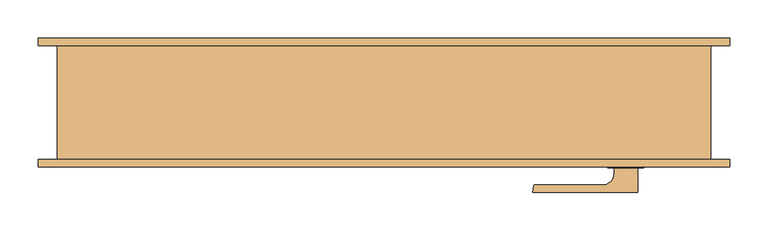
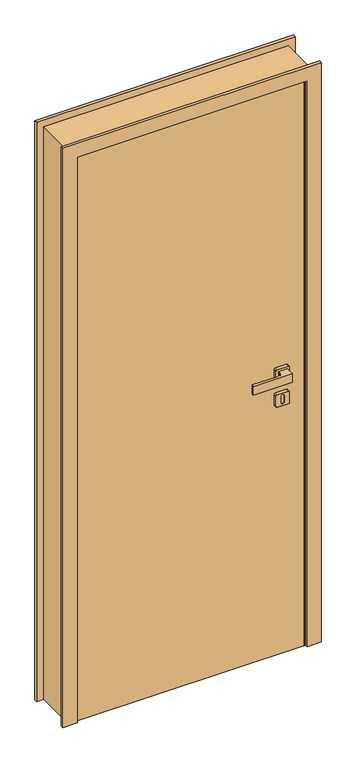
"""IFC4 building model written with IfcOpenShell, lengths in millimetres: door geometry, porta multiplas_growarq : porta giro simples 80 cm_growarq 2."""

from ifc_helpers import new_model, si_unit, point, frame, frame_2d, origin, origin_with_axes, place, context, project, spatial, polyline, circle_curve, trimmed, segment, composite_curve, outline, extrude, source, transform, mapped, element, save
from ifc_brep_helpers import plane_surface, cylinder_surface, revolved_surface, advanced_brep


def door_ea212285(model_context):
    return source(origin(), model_context, "Body", "SolidModel", [
        advanced_brep(
        [(337.5247906, -86.0, 975.2140175), (298.4820692, -86.0, 975.2140175), (294.475196, -86.0, 971.2071442), (294.475196, -86.0, 932.3348635), (298.475196, -86.0, 928.3348635), (337.5247906, -86.0, 928.3348635), (341.5247906, -86.0, 932.3348635), (341.5247906, -86.0, 971.2140175), (323.0036235, -86.0, 963.1453546), (323.0036235, -86.0, 940.4035264), (312.9935514, -86.0, 940.4035264), (312.9935514, -86.0, 963.1453546), (337.5247906, -75.0, 975.2140175), (341.5247906, -75.0, 971.2140175), (341.5247906, -75.0, 932.3348635), (337.5247906, -75.0, 928.3348635), (298.475196, -75.0, 928.3348635), (294.475196, -75.0, 932.3348635), (294.475196, -75.0, 971.2071442), (298.4820692, -75.0, 975.2140175), (323.0036235, -84.0, 940.4035264), (323.0036235, -84.0, 963.1453546), (312.9935514, -84.0, 963.1453546), (312.9935514, -84.0, 940.4035264)],
        [
            (0, 1),
            (1, 2, circle_curve(frame((298.4820692, -86.0, 971.2071442), z_axis=(0.0, -1.0, 0.0), x_axis=(1.0, 0.0, 0.0)), 4.0068732)),
            (2, 3),
            (3, 4, circle_curve(frame((298.475196, -86.0, 932.3348635), z_axis=(0.0, -1.0, 0.0), x_axis=(1.0, 0.0, 0.0)), 4.0)),
            (4, 5),
            (5, 6, circle_curve(frame((337.5247906, -86.0, 932.3348635), z_axis=(0.0, -1.0, 0.0), x_axis=(1.0, 0.0, 0.0)), 4.0)),
            (6, 7),
            (7, 0, circle_curve(frame((337.5247906, -86.0, 971.2140175), z_axis=(0.0, -1.0, 0.0), x_axis=(1.0, 0.0, 0.0)), 4.0)),
            (8, 9),
            (9, 10, circle_curve(frame((317.9985874, -86.0, 940.4035264), z_axis=(0.0, 1.0, 0.0), x_axis=(1.0, 0.0, 0.0)), 5.0050361)),
            (10, 11),
            (11, 8, circle_curve(frame((317.9985874, -86.0, 963.1453546), z_axis=(0.0, 1.0, 0.0), x_axis=(1.0, 0.0, 0.0)), 5.0050361)),
            (12, 13, circle_curve(frame((337.5247906, -75.0, 971.2140175), z_axis=(0.0, 1.0, 0.0), x_axis=(1.0, 0.0, 0.0)), 4.0)),
            (13, 14),
            (14, 15, circle_curve(frame((337.5247906, -75.0, 932.3348635), z_axis=(0.0, 1.0, 0.0), x_axis=(1.0, 0.0, 0.0)), 4.0)),
            (15, 16),
            (16, 17, circle_curve(frame((298.475196, -75.0, 932.3348635), z_axis=(0.0, 1.0, 0.0), x_axis=(1.0, 0.0, 0.0)), 4.0)),
            (17, 18),
            (18, 19, circle_curve(frame((298.4820692, -75.0, 971.2071442), z_axis=(0.0, 1.0, 0.0), x_axis=(1.0, 0.0, 0.0)), 4.0068732)),
            (19, 12),
            (0, 12),
            (19, 1),
            (18, 2),
            (17, 3),
            (16, 4),
            (15, 5),
            (14, 6),
            (13, 7),
            (20, 21),
            (21, 22, circle_curve(frame((317.9985874, -84.0, 963.1453546), z_axis=(0.0, -1.0, 0.0), x_axis=(1.0, 0.0, 0.0)), 5.0050361)),
            (22, 23),
            (23, 20, circle_curve(frame((317.9985874, -84.0, 940.4035264), z_axis=(0.0, -1.0, 0.0), x_axis=(1.0, 0.0, 0.0)), 5.0050361)),
            (20, 9),
            (8, 21),
            (22, 11),
            (10, 23),
        ],
        [
            plane_surface(frame((298.4781039, -86.0, 975.2140175), z_axis=(0.0, -1.0, 0.0), x_axis=(-1.0, 0.0, 0.0))),
            plane_surface(frame((298.4781039, -75.0, 975.2140175), z_axis=(0.0, 1.0, 0.0), x_axis=(1.0, 0.0, 0.0))),
            plane_surface(frame((337.5247906, -86.0, 975.2140175), z_axis=(0.0, 0.0, 1.0), x_axis=(0.0, 1.0, 0.0))),
            cylinder_surface(frame((298.4820692, -75.0, 971.2071442), z_axis=(0.0, -1.0, 0.0), x_axis=(1.0, 0.0, 0.0)), 4.0068732),
            plane_surface(frame((294.475196, -86.0, 971.2071442), z_axis=(-1.0, 0.0, 0.0), x_axis=(0.0, 1.0, 0.0))),
            cylinder_surface(frame((298.475196, -75.0, 932.3348635), z_axis=(0.0, -1.0, 0.0), x_axis=(1.0, 0.0, 0.0)), 4.0),
            plane_surface(frame((298.475196, -86.0, 928.3348635), z_axis=(0.0, 0.0, -1.0), x_axis=(0.0, 1.0, 0.0))),
            cylinder_surface(frame((337.5247906, -75.0, 932.3348635), z_axis=(0.0, -1.0, 0.0), x_axis=(1.0, 0.0, 0.0)), 4.0),
            plane_surface(frame((341.5247906, -86.0, 932.3348635), z_axis=(1.0, 0.0, 0.0), x_axis=(0.0, 1.0, 0.0))),
            cylinder_surface(frame((337.5247906, -75.0, 971.2140175), z_axis=(0.0, -1.0, 0.0), x_axis=(1.0, 0.0, 0.0)), 4.0),
            plane_surface(frame((323.0036235, -84.0, 952.9958878), z_axis=(0.0, -1.0, 0.0), x_axis=(0.0, 0.0, -1.0))),
            plane_surface(frame((323.0036235, -86.0, 940.4035264), z_axis=(-1.0, 0.0, 0.0), x_axis=(0.0, 1.0, 0.0))),
            plane_surface(frame((312.9935514, -86.0, 963.1453546), z_axis=(1.0, 0.0, 0.0), x_axis=(0.0, 1.0, 0.0))),
            revolved_surface(polyline([(323.0036235, -86.0, 940.4035264), (323.0036235, -84.0, 940.4035264)]), (317.9985874, -84.0, 940.4035264), (0.0, -1.0, 0.0)),
            revolved_surface(polyline([(323.0036235, -86.0, 963.1453546), (323.0036235, -84.0, 963.1453546)]), (317.9985874, -84.0, 963.1453546), (0.0, -1.0, 0.0)),
        ],
        [
            (0, [[1, 2, 3, 4, 5, 6, 7, 8], [9, 10, 11, 12]]),
            (1, [[13, 14, 15, 16, 17, 18, 19, 20]]),
            (2, [[-1, 21, -20, 22]]),
            (3, [[-2, -22, -19, 23]]),
            (4, [[-3, -23, -18, 24]]),
            (5, [[-4, -24, -17, 25]]),
            (6, [[-5, -25, -16, 26]]),
            (7, [[-6, -26, -15, 27]]),
            (8, [[-7, -27, -14, 28]]),
            (9, [[-8, -28, -13, -21]]),
            (10, [[29, 30, 31, 32]]),
            (11, [[-29, 33, -9, 34]]),
            (12, [[-31, 35, -11, 36]]),
            (13, [[-32, -36, -10, -33]]),
            (14, [[-30, -34, -12, -35]]),
        ],
    ),
        advanced_brep(
        [(337.5247906, -86.0, 1068.227973), (298.4820692, -86.0, 1068.227973), (294.475196, -86.0, 1064.2210998), (294.475196, -86.0, 1025.3488191), (298.475196, -86.0, 1021.3488191), (337.5247906, -86.0, 1021.3488191), (341.5247906, -86.0, 1025.3488191), (341.5247906, -86.0, 1064.227973), (337.5247906, -75.0, 1068.227973), (341.5247906, -75.0, 1064.227973), (341.5247906, -75.0, 1025.3488191), (337.5247906, -75.0, 1021.3488191), (298.475196, -75.0, 1021.3488191), (294.475196, -75.0, 1025.3488191), (294.475196, -75.0, 1064.2210998), (298.4820692, -75.0, 1068.227973)],
        [
            (0, 1),
            (1, 2, circle_curve(frame((298.4820692, -86.0, 1064.2210998), z_axis=(0.0, -1.0, 0.0), x_axis=(1.0, 0.0, 0.0)), 4.0068732)),
            (2, 3),
            (3, 4, circle_curve(frame((298.475196, -86.0, 1025.3488191), z_axis=(0.0, -1.0, 0.0), x_axis=(1.0, 0.0, 0.0)), 4.0)),
            (4, 5),
            (5, 6, circle_curve(frame((337.5247906, -86.0, 1025.3488191), z_axis=(0.0, -1.0, 0.0), x_axis=(1.0, 0.0, 0.0)), 4.0)),
            (6, 7),
            (7, 0, circle_curve(frame((337.5247906, -86.0, 1064.227973), z_axis=(0.0, -1.0, 0.0), x_axis=(1.0, 0.0, 0.0)), 4.0)),
            (8, 9, circle_curve(frame((337.5247906, -75.0, 1064.227973), z_axis=(0.0, 1.0, 0.0), x_axis=(1.0, 0.0, 0.0)), 4.0)),
            (9, 10),
            (10, 11, circle_curve(frame((337.5247906, -75.0, 1025.3488191), z_axis=(0.0, 1.0, 0.0), x_axis=(1.0, 0.0, 0.0)), 4.0)),
            (11, 12),
            (12, 13, circle_curve(frame((298.475196, -75.0, 1025.3488191), z_axis=(0.0, 1.0, 0.0), x_axis=(1.0, 0.0, 0.0)), 4.0)),
            (13, 14),
            (14, 15, circle_curve(frame((298.4820692, -75.0, 1064.2210998), z_axis=(0.0, 1.0, 0.0), x_axis=(1.0, 0.0, 0.0)), 4.0068732)),
            (15, 8),
            (0, 8),
            (15, 1),
            (14, 2),
            (13, 3),
            (12, 4),
            (11, 5),
            (10, 6),
            (9, 7),
        ],
        [
            plane_surface(frame((298.4781039, -86.0, 975.2140175), z_axis=(0.0, -1.0, 0.0), x_axis=(-1.0, 0.0, 0.0))),
            plane_surface(frame((298.4781039, -75.0, 975.2140175), z_axis=(0.0, 1.0, 0.0), x_axis=(1.0, 0.0, 0.0))),
            plane_surface(frame((337.5247906, -86.0, 1068.227973), z_axis=(0.0, 0.0, 1.0), x_axis=(0.0, 1.0, 0.0))),
            cylinder_surface(frame((298.4820692, -75.0, 1064.2210998), z_axis=(0.0, -1.0, 0.0), x_axis=(1.0, 0.0, 0.0)), 4.0068732),
            plane_surface(frame((294.475196, -86.0, 1064.2210998), z_axis=(-1.0, 0.0, 0.0), x_axis=(0.0, 1.0, 0.0))),
            cylinder_surface(frame((298.475196, -75.0, 1025.3488191), z_axis=(0.0, -1.0, 0.0), x_axis=(1.0, 0.0, 0.0)), 4.0),
            plane_surface(frame((298.475196, -86.0, 1021.3488191), z_axis=(0.0, 0.0, -1.0), x_axis=(0.0, 1.0, 0.0))),
            cylinder_surface(frame((337.5247906, -75.0, 1025.3488191), z_axis=(0.0, -1.0, 0.0), x_axis=(1.0, 0.0, 0.0)), 4.0),
            plane_surface(frame((341.5247906, -86.0, 1025.3488191), z_axis=(1.0, 0.0, 0.0), x_axis=(0.0, 1.0, 0.0))),
            cylinder_surface(frame((337.5247906, -75.0, 1064.227973), z_axis=(0.0, -1.0, 0.0), x_axis=(1.0, 0.0, 0.0)), 4.0),
        ],
        [
            (0, [[1, 2, 3, 4, 5, 6, 7, 8]]),
            (1, [[9, 10, 11, 12, 13, 14, 15, 16]]),
            (2, [[-1, 17, -16, 18]]),
            (3, [[-2, -18, -15, 19]]),
            (4, [[-3, -19, -14, 20]]),
            (5, [[-4, -20, -13, 21]]),
            (6, [[-5, -21, -12, 22]]),
            (7, [[-6, -22, -11, 23]]),
            (8, [[-7, -23, -10, 24]]),
            (9, [[-8, -24, -9, -17]]),
        ],
    ),
        extrude(outline(composite_curve([segment(polyline([(333.5247906, -118.5150355), (195.5657525, -118.5150355), (197.1621392, -109.4614767)]), True, "CONTINUOUS"), segment(trimmed(circle_curve(frame_2d((198.1590205, -109.6372538)), 1.0122598), [point((197.1621392, -109.4614767))], [point((198.1590205, -108.6249939))], False, "CARTESIAN"), True, "CONTINUOUS"), segment(polyline([(198.1590205, -108.6249939), (287.4483579, -108.6249939)]), True, "CONTINUOUS"), segment(trimmed(circle_curve(frame_2d((287.4483579, -93.5981558)), 15.0268381), [point((287.4483579, -108.6249939))], [point((302.475196, -93.5981558))], True, "CARTESIAN"), True, "CONTINUOUS"), segment(polyline([(302.475196, -93.5981558), (302.475196, -86.7793682), (333.5247906, -86.7793682), (333.5247906, -118.5150355)]), True, "CONTINUOUS")], self_intersect=False)), frame((0.0, 0.0, 1029.3488191), z_axis=(0.0, 0.0, 1.0), x_axis=(1.0, 0.0, 0.0)), (0.0, 0.0, 1.0), 30.8791539),
        advanced_brep(
        [(337.5247906, -34.0, 975.2140175), (341.5247906, -34.0, 971.2140175), (341.5247906, -34.0, 932.3348635), (337.5247906, -34.0, 928.3348635), (298.475196, -34.0, 928.3348635), (294.475196, -34.0, 932.3348635), (294.475196, -34.0, 971.2071442), (298.4820692, -34.0, 975.2140175), (323.0036235, -34.0, 963.1453546), (312.9935514, -34.0, 963.1453546), (312.9935514, -34.0, 940.4035264), (323.0036235, -34.0, 940.4035264), (337.5247906, -45.0, 975.2140175), (298.4820692, -45.0, 975.2140175), (294.475196, -45.0, 971.2071442), (294.475196, -45.0, 932.3348635), (298.475196, -45.0, 928.3348635), (337.5247906, -45.0, 928.3348635), (341.5247906, -45.0, 932.3348635), (341.5247906, -45.0, 971.2140175), (323.0036235, -36.0, 940.4035264), (312.9935514, -36.0, 940.4035264), (312.9935514, -36.0, 963.1453546), (323.0036235, -36.0, 963.1453546)],
        [
            (0, 1, circle_curve(frame((337.5247906, -34.0, 971.2140175), z_axis=(0.0, 1.0, 0.0), x_axis=(1.0, 0.0, 0.0)), 4.0)),
            (1, 2),
            (2, 3, circle_curve(frame((337.5247906, -34.0, 932.3348635), z_axis=(0.0, 1.0, 0.0), x_axis=(1.0, 0.0, 0.0)), 4.0)),
            (3, 4),
            (4, 5, circle_curve(frame((298.475196, -34.0, 932.3348635), z_axis=(0.0, 1.0, 0.0), x_axis=(1.0, 0.0, 0.0)), 4.0)),
            (5, 6),
            (6, 7, circle_curve(frame((298.4820692, -34.0, 971.2071442), z_axis=(0.0, 1.0, 0.0), x_axis=(1.0, 0.0, 0.0)), 4.0068732)),
            (7, 0),
            (8, 9, circle_curve(frame((317.9985874, -34.0, 963.1453546), z_axis=(0.0, -1.0, 0.0), x_axis=(1.0, 0.0, 0.0)), 5.0050361)),
            (9, 10),
            (10, 11, circle_curve(frame((317.9985874, -34.0, 940.4035264), z_axis=(0.0, -1.0, 0.0), x_axis=(1.0, 0.0, 0.0)), 5.0050361)),
            (11, 8),
            (12, 13),
            (13, 14, circle_curve(frame((298.4820692, -45.0, 971.2071442), z_axis=(0.0, -1.0, 0.0), x_axis=(1.0, 0.0, 0.0)), 4.0068732)),
            (14, 15),
            (15, 16, circle_curve(frame((298.475196, -45.0, 932.3348635), z_axis=(0.0, -1.0, 0.0), x_axis=(1.0, 0.0, 0.0)), 4.0)),
            (16, 17),
            (17, 18, circle_curve(frame((337.5247906, -45.0, 932.3348635), z_axis=(0.0, -1.0, 0.0), x_axis=(1.0, 0.0, 0.0)), 4.0)),
            (18, 19),
            (19, 12, circle_curve(frame((337.5247906, -45.0, 971.2140175), z_axis=(0.0, -1.0, 0.0), x_axis=(1.0, 0.0, 0.0)), 4.0)),
            (7, 13),
            (12, 0),
            (6, 14),
            (5, 15),
            (4, 16),
            (3, 17),
            (2, 18),
            (1, 19),
            (20, 21, circle_curve(frame((317.9985874, -36.0, 940.4035264), z_axis=(0.0, 1.0, 0.0), x_axis=(1.0, 0.0, 0.0)), 5.0050361)),
            (21, 22),
            (22, 23, circle_curve(frame((317.9985874, -36.0, 963.1453546), z_axis=(0.0, 1.0, 0.0), x_axis=(1.0, 0.0, 0.0)), 5.0050361)),
            (23, 20),
            (23, 8),
            (11, 20),
            (21, 10),
            (9, 22),
        ],
        [
            plane_surface(frame((298.4781039, -34.0, 975.2140175), z_axis=(0.0, 1.0, 0.0), x_axis=(-1.0, 0.0, 0.0))),
            plane_surface(frame((298.4781039, -45.0, 975.2140175), z_axis=(0.0, -1.0, 0.0), x_axis=(1.0, 0.0, 0.0))),
            plane_surface(frame((337.5247906, -34.0, 975.2140175), z_axis=(0.0, 0.0, 1.0), x_axis=(0.0, -1.0, 0.0))),
            cylinder_surface(frame((298.4820692, -45.0, 971.2071442), z_axis=(0.0, 1.0, 0.0), x_axis=(1.0, 0.0, 0.0)), 4.0068732),
            plane_surface(frame((294.475196, -34.0, 971.2071442), z_axis=(-1.0, 0.0, 0.0), x_axis=(0.0, -1.0, 0.0))),
            cylinder_surface(frame((298.475196, -45.0, 932.3348635), z_axis=(0.0, 1.0, 0.0), x_axis=(1.0, 0.0, 0.0)), 4.0),
            plane_surface(frame((298.475196, -34.0, 928.3348635), z_axis=(0.0, 0.0, -1.0), x_axis=(0.0, -1.0, 0.0))),
            cylinder_surface(frame((337.5247906, -45.0, 932.3348635), z_axis=(0.0, 1.0, 0.0), x_axis=(1.0, 0.0, 0.0)), 4.0),
            plane_surface(frame((341.5247906, -34.0, 932.3348635), z_axis=(1.0, 0.0, 0.0), x_axis=(0.0, -1.0, 0.0))),
            cylinder_surface(frame((337.5247906, -45.0, 971.2140175), z_axis=(0.0, 1.0, 0.0), x_axis=(1.0, 0.0, 0.0)), 4.0),
            plane_surface(frame((323.0036235, -36.0, 952.9958878), z_axis=(0.0, 1.0, 0.0), x_axis=(0.0, 0.0, -1.0))),
            plane_surface(frame((323.0036235, -34.0, 940.4035264), z_axis=(-1.0, 0.0, 0.0), x_axis=(0.0, -1.0, 0.0))),
            plane_surface(frame((312.9935514, -34.0, 963.1453546), z_axis=(1.0, 0.0, 0.0), x_axis=(0.0, -1.0, 0.0))),
            revolved_surface(polyline([(323.0036235, -34.0, 940.4035264), (323.0036235, -36.0, 940.4035264)]), (317.9985874, -36.0, 940.4035264), (0.0, 1.0, 0.0)),
            revolved_surface(polyline([(323.0036235, -34.0, 963.1453546), (323.0036235, -36.0, 963.1453546)]), (317.9985874, -36.0, 963.1453546), (0.0, 1.0, 0.0)),
        ],
        [
            (0, [[1, 2, 3, 4, 5, 6, 7, 8], [9, 10, 11, 12]]),
            (1, [[13, 14, 15, 16, 17, 18, 19, 20]]),
            (2, [[21, -13, 22, -8]]),
            (3, [[23, -14, -21, -7]]),
            (4, [[24, -15, -23, -6]]),
            (5, [[25, -16, -24, -5]]),
            (6, [[26, -17, -25, -4]]),
            (7, [[27, -18, -26, -3]]),
            (8, [[28, -19, -27, -2]]),
            (9, [[-22, -20, -28, -1]]),
            (10, [[29, 30, 31, 32]]),
            (11, [[33, -12, 34, -32]]),
            (12, [[35, -10, 36, -30]]),
            (13, [[-34, -11, -35, -29]]),
            (14, [[-36, -9, -33, -31]]),
        ],
    ),
        advanced_brep(
        [(337.5247906, -34.0, 1068.227973), (341.5247906, -34.0, 1064.227973), (341.5247906, -34.0, 1025.3488191), (337.5247906, -34.0, 1021.3488191), (298.475196, -34.0, 1021.3488191), (294.475196, -34.0, 1025.3488191), (294.475196, -34.0, 1064.2210998), (298.4820692, -34.0, 1068.227973), (337.5247906, -45.0, 1068.227973), (298.4820692, -45.0, 1068.227973), (294.475196, -45.0, 1064.2210998), (294.475196, -45.0, 1025.3488191), (298.475196, -45.0, 1021.3488191), (337.5247906, -45.0, 1021.3488191), (341.5247906, -45.0, 1025.3488191), (341.5247906, -45.0, 1064.227973)],
        [
            (0, 1, circle_curve(frame((337.5247906, -34.0, 1064.227973), z_axis=(0.0, 1.0, 0.0), x_axis=(1.0, 0.0, 0.0)), 4.0)),
            (1, 2),
            (2, 3, circle_curve(frame((337.5247906, -34.0, 1025.3488191), z_axis=(0.0, 1.0, 0.0), x_axis=(1.0, 0.0, 0.0)), 4.0)),
            (3, 4),
            (4, 5, circle_curve(frame((298.475196, -34.0, 1025.3488191), z_axis=(0.0, 1.0, 0.0), x_axis=(1.0, 0.0, 0.0)), 4.0)),
            (5, 6),
            (6, 7, circle_curve(frame((298.4820692, -34.0, 1064.2210998), z_axis=(0.0, 1.0, 0.0), x_axis=(1.0, 0.0, 0.0)), 4.0068732)),
            (7, 0),
            (8, 9),
            (9, 10, circle_curve(frame((298.4820692, -45.0, 1064.2210998), z_axis=(0.0, -1.0, 0.0), x_axis=(1.0, 0.0, 0.0)), 4.0068732)),
            (10, 11),
            (11, 12, circle_curve(frame((298.475196, -45.0, 1025.3488191), z_axis=(0.0, -1.0, 0.0), x_axis=(1.0, 0.0, 0.0)), 4.0)),
            (12, 13),
            (13, 14, circle_curve(frame((337.5247906, -45.0, 1025.3488191), z_axis=(0.0, -1.0, 0.0), x_axis=(1.0, 0.0, 0.0)), 4.0)),
            (14, 15),
            (15, 8, circle_curve(frame((337.5247906, -45.0, 1064.227973), z_axis=(0.0, -1.0, 0.0), x_axis=(1.0, 0.0, 0.0)), 4.0)),
            (7, 9),
            (8, 0),
            (6, 10),
            (5, 11),
            (4, 12),
            (3, 13),
            (2, 14),
            (1, 15),
        ],
        [
            plane_surface(frame((298.4781039, -34.0, 975.2140175), z_axis=(0.0, 1.0, 0.0), x_axis=(-1.0, 0.0, 0.0))),
            plane_surface(frame((298.4781039, -45.0, 975.2140175), z_axis=(0.0, -1.0, 0.0), x_axis=(1.0, 0.0, 0.0))),
            plane_surface(frame((337.5247906, -34.0, 1068.227973), z_axis=(0.0, 0.0, 1.0), x_axis=(0.0, -1.0, 0.0))),
            cylinder_surface(frame((298.4820692, -45.0, 1064.2210998), z_axis=(0.0, 1.0, 0.0), x_axis=(1.0, 0.0, 0.0)), 4.0068732),
            plane_surface(frame((294.475196, -34.0, 1064.2210998), z_axis=(-1.0, 0.0, 0.0), x_axis=(0.0, -1.0, 0.0))),
            cylinder_surface(frame((298.475196, -45.0, 1025.3488191), z_axis=(0.0, 1.0, 0.0), x_axis=(1.0, 0.0, 0.0)), 4.0),
            plane_surface(frame((298.475196, -34.0, 1021.3488191), z_axis=(0.0, 0.0, -1.0), x_axis=(0.0, -1.0, 0.0))),
            cylinder_surface(frame((337.5247906, -45.0, 1025.3488191), z_axis=(0.0, 1.0, 0.0), x_axis=(1.0, 0.0, 0.0)), 4.0),
            plane_surface(frame((341.5247906, -34.0, 1025.3488191), z_axis=(1.0, 0.0, 0.0), x_axis=(0.0, -1.0, 0.0))),
            cylinder_surface(frame((337.5247906, -45.0, 1064.227973), z_axis=(0.0, 1.0, 0.0), x_axis=(1.0, 0.0, 0.0)), 4.0),
        ],
        [
            (0, [[1, 2, 3, 4, 5, 6, 7, 8]]),
            (1, [[9, 10, 11, 12, 13, 14, 15, 16]]),
            (2, [[17, -9, 18, -8]]),
            (3, [[19, -10, -17, -7]]),
            (4, [[20, -11, -19, -6]]),
            (5, [[21, -12, -20, -5]]),
            (6, [[22, -13, -21, -4]]),
            (7, [[23, -14, -22, -3]]),
            (8, [[24, -15, -23, -2]]),
            (9, [[-18, -16, -24, -1]]),
        ],
    ),
        extrude(outline(composite_curve([segment(polyline([(333.5247906, -1.4849645), (333.5247906, -33.2206318), (302.475196, -33.2206318), (302.475196, -26.4018442)]), True, "CONTINUOUS"), segment(trimmed(circle_curve(frame_2d((287.4483579, -26.4018442)), 15.0268381), [point((302.475196, -26.4018442))], [point((287.4483579, -11.3750061))], True, "CARTESIAN"), True, "CONTINUOUS"), segment(polyline([(287.4483579, -11.3750061), (198.1590205, -11.3750061)]), True, "CONTINUOUS"), segment(trimmed(circle_curve(frame_2d((198.1590205, -10.3627462)), 1.0122598), [point((198.1590205, -11.3750061))], [point((197.1621392, -10.5385233))], False, "CARTESIAN"), True, "CONTINUOUS"), segment(polyline([(197.1621392, -10.5385233), (195.5657525, -1.4849645), (333.5247906, -1.4849645)]), True, "CONTINUOUS")], self_intersect=False)), frame((0.0, 0.0, 1029.3488191), z_axis=(0.0, 0.0, 1.0), x_axis=(1.0, 0.0, 0.0)), (0.0, 0.0, 1.0), 30.8791539),
        extrude(outline(polyline([(398.0, -45.0), (398.0, -75.0), (-398.0, -75.0), (-398.0, -45.0), (398.0, -45.0)])), origin_with_axes(), (0.0, 0.0, 1.0), 2098.0),
        extrude(outline(polyline([(0.0, 400.0), (0.0, 430.0), (2130.0, 430.0), (2130.0, -430.0), (0.0, -430.0), (0.0, -400.0), (2100.0, -400.0), (2100.0, 400.0), (0.0, 400.0)])), frame((0.0, -75.0, 0.0), z_axis=(0.0, 1.0, 0.0), x_axis=(0.0, 0.0, 1.0)), (0.0, 0.0, 1.0), 150.0),
        extrude(outline(polyline([(2155.0, -455.0), (0.0, -455.0), (0.0, -405.0), (2105.0, -405.0), (2105.0, 405.0), (0.0, 405.0), (0.0, 455.0), (2155.0, 455.0), (2155.0, -455.0)])), frame((0.0, 75.0, 0.0), z_axis=(0.0, 1.0, 0.0), x_axis=(0.0, 0.0, 1.0)), (0.0, 0.0, 1.0), 10.0),
        extrude(outline(polyline([(2105.0, 405.0), (0.0, 405.0), (0.0, 455.0), (2155.0, 455.0), (2155.0, -455.0), (0.0, -455.0), (0.0, -405.0), (2105.0, -405.0), (2105.0, 405.0)])), frame((0.0, -85.0, 0.0), z_axis=(0.0, 1.0, 0.0), x_axis=(0.0, 0.0, 1.0)), (0.0, 0.0, 1.0), 10.0),
    ])


if __name__ == "__main__":
    model = new_model("IFC4")
    model_context = context("Model", 3, world=origin())
    ifc_project = project(units=[si_unit("LENGTHUNIT", "METRE", prefix="MILLI")], contexts=[model_context])
    site = spatial("IfcSite", under=ifc_project)
    building = spatial("IfcBuilding", under=site)
    placement = place(None, origin())
    door_shape = door_ea212285(model_context)
    element("IfcDoor", 1, ObjectType="porta multiplas_growarq : porta giro simples 80 cm_growarq 2", at=placement, inside=building, context=model_context, shape_type="MappedRepresentation", body=[
        mapped(door_shape, transform((0.0, 0.0, 0.0), x_axis=(1.0, 0.0, 0.0), y_axis=(0.0, 1.0, 0.0), z_axis=(0.0, 0.0, 1.0))),
    ])
    save(model, "model.ifc")

# Revit data of these elements
# Type "porta multiplas_growarq : porta giro simples 80 cm_growarq 2"
#   Type Mark = "C39"
#   Description = "Porta de Madeira com uma folha de abrir"
#   Analytic Construction = "<None>"
#   Rough Width = 860 mm
#   Largura Guarnição = 50 mm
#   Espessura Guarnição = 10 mm
#   Thickness = 30 mm
#   Rough Height = 2130 mm
#   Marco = 30 mm
#   Largura Folha Eixo = 596 mm
#   Height = 2100 mm
#   Width = 800 mm
#   Largura Folha = 796 mm
#   Eixo = 200 mm
#   Altura Folha = 2098 mm
#   Abertura correr [instance default] = 200 mm
#   Abertura [instance default] = 0.00°
#   Simples = yes
#   Guarnição = yes
#   Eixo Folha = no
#   Dupla = no
#   Correr = no
#   Material = .pintura preta_growarq
#   Function = (empty or 0)
#   Wall Closure = (empty or 0)
# Element 1 (IfcDoor, "porta multiplas_growarq : porta giro simples 80 cm_growarq 2")
#   Materials on its faces: ".pintura preta_growarq"
# Materials
#   ".pintura preta_growarq": class "Pintura", colour RGB 30 30 30, transparency 0, Description = "Pintura preta", Cost = 0
